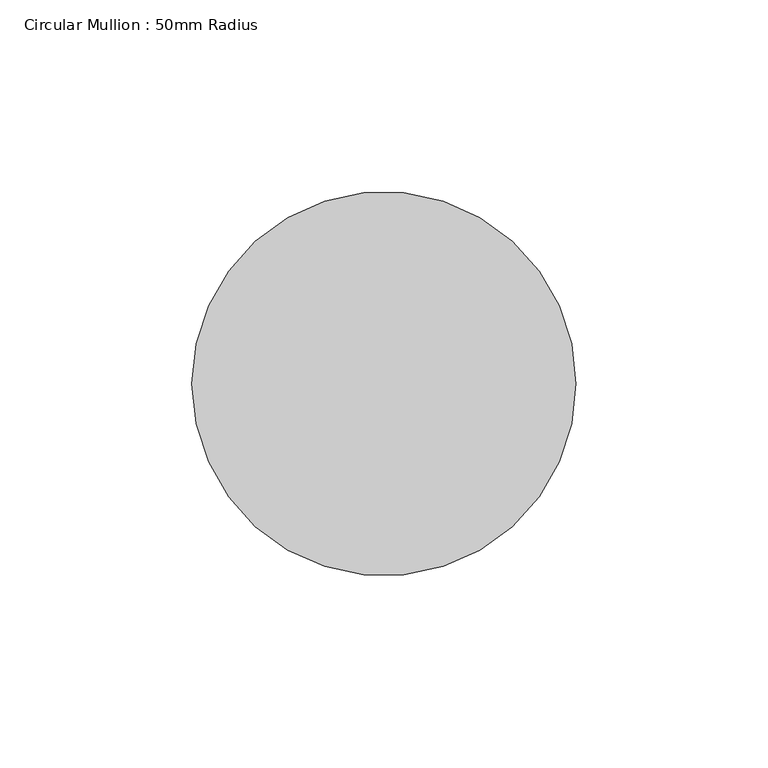
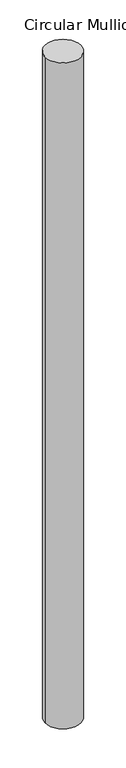
"""IFC4 building model written with IfcOpenShell, lengths in millimetres: member geometry, Circular Mullion : 50mm Radius."""

from ifc_helpers import new_model, si_unit, point, frame, frame_2d, origin, place, context, project, spatial, circle_curve, trimmed, segment, composite_curve, outline, extrude, source, transform, mapped, element, save


def circular_mullion_50mm_radius_e48f73f0(model_context):
    return source(origin(), model_context, "Body", "SweptSolid", [
        extrude(outline(composite_curve([segment(trimmed(circle_curve(frame_2d((-50.0, 0.0)), 50.0), [point((0.0, 0.0))], [point((-100.0, 0.0))], False, "CARTESIAN"), True, "CONTINUOUS"), segment(trimmed(circle_curve(frame_2d((-50.0, 0.0)), 50.0), [point((-100.0, 0.0))], [point((0.0, 0.0))], False, "CARTESIAN"), True, "CONTINUOUS")], self_intersect=False)), frame((0.0, 0.0, -1966.3350845), z_axis=(0.0, 0.0, 1.0), x_axis=(1.0, 0.0, 0.0)), (0.0, 0.0, 1.0), 1966.3350845),
    ])


if __name__ == "__main__":
    model = new_model("IFC4")
    model_context = context("Model", 3, world=origin())
    ifc_project = project(units=[si_unit("LENGTHUNIT", "METRE", prefix="MILLI")], contexts=[model_context])
    site = spatial("IfcSite", under=ifc_project)
    building = spatial("IfcBuilding", under=site)
    placement = place(None, origin())
    circular_mullion_50mm_radius_shape = circular_mullion_50mm_radius_e48f73f0(model_context)
    element("IfcMember", 1, ObjectType="Circular Mullion : 50mm Radius", at=placement, inside=building, context=model_context, shape_type="MappedRepresentation", body=[
        mapped(circular_mullion_50mm_radius_shape, transform((0.0, 0.0, 0.0), x_axis=(1.0, 0.0, 0.0), y_axis=(0.0, 1.0, 0.0), z_axis=(0.0, 0.0, 1.0))),
    ])
    save(model, "model.ifc")

# Revit data of these elements
# Type "Circular Mullion : 50mm Radius"
#   built-in parameter 1007350 = 0.164042 (stored number, unit not read)
# Element 1 (IfcMember, "Circular Mullion : 50mm Radius")
#   Materials on its faces: "Aluminium"
# Materials
#   "Aluminium": class "Metal", colour RGB 247 247 247, transparency 0, Description = "Aluminium 6061", Cost = 0
